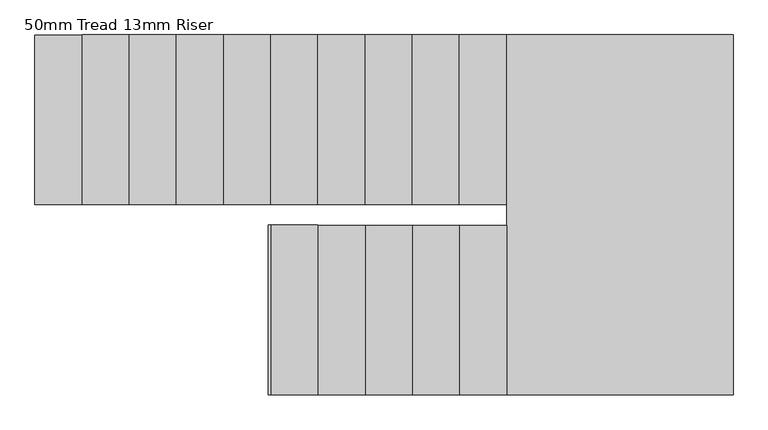
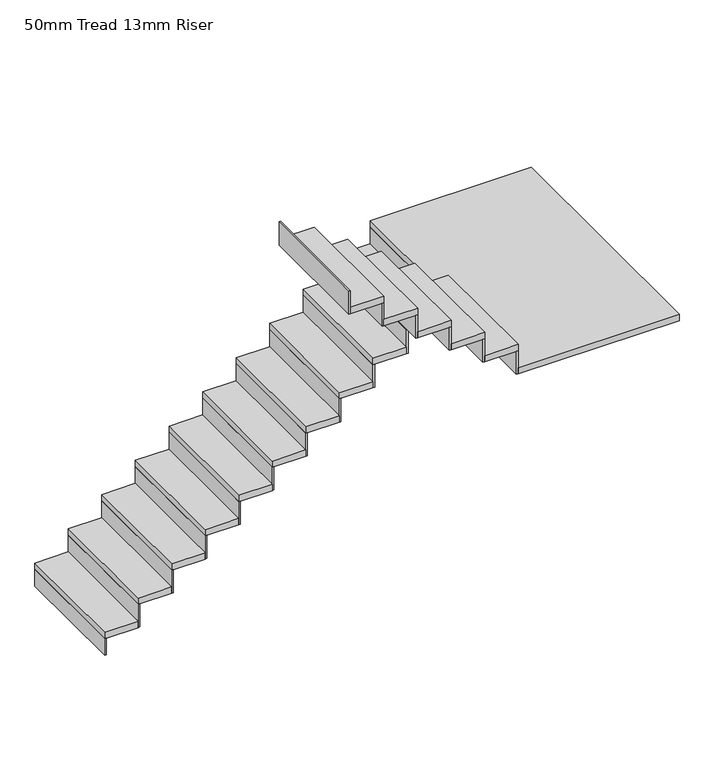
"""IFC4 building model written with IfcOpenShell, lengths in millimetres: stair flight geometry, 50mm Tread 13mm Riser."""

from ifc_helpers import new_model, si_unit, frame, origin, place, context, project, spatial, polyline, outline, extrude, source, transform, mapped, element, save


def stair_flight_50mm_tread_13mm_riser_aed1185b(model_context):
    return source(origin(), model_context, "Body", "SweptSolid", [
        extrude(outline(polyline([(-8706.7253352, 6708.2914588), (-8719.2253352, 6708.2914588), (-8719.2253352, 7608.2914588), (-8706.7253352, 7608.2914588), (-8706.7253352, 6708.2914588)])), frame((0.0, 0.0, 450.0), z_axis=(0.0, 0.0, 1.0), x_axis=(1.0, 0.0, 0.0)), (0.0, 0.0, 1.0), 132.3529412),
        extrude(outline(polyline([(-8469.2253352, 7608.2914588), (-8469.2253352, 6708.2914588), (-8719.2253352, 6708.2914588), (-8719.2253352, 7608.2914588), (-8469.2253352, 7608.2914588)])), frame((0.0, 0.0, 582.3529412), z_axis=(0.0, 0.0, 1.0), x_axis=(1.0, 0.0, 0.0)), (0.0, 0.0, 1.0), 50.0),
        extrude(outline(polyline([(-8456.7253352, 6708.2914588), (-8469.2253352, 6708.2914588), (-8469.2253352, 7608.2914588), (-8456.7253352, 7608.2914588), (-8456.7253352, 6708.2914588)])), frame((0.0, 0.0, 582.3529412), z_axis=(0.0, 0.0, 1.0), x_axis=(1.0, 0.0, 0.0)), (0.0, 0.0, 1.0), 182.3529412),
        extrude(outline(polyline([(-8219.2253352, 7608.2914588), (-8219.2253352, 6708.2914588), (-8469.2253352, 6708.2914588), (-8469.2253352, 7608.2914588), (-8219.2253352, 7608.2914588)])), frame((0.0, 0.0, 764.7058824), z_axis=(0.0, 0.0, 1.0), x_axis=(1.0, 0.0, 0.0)), (0.0, 0.0, 1.0), 50.0),
        extrude(outline(polyline([(-8206.7253352, 6708.2914588), (-8219.2253352, 6708.2914588), (-8219.2253352, 7608.2914588), (-8206.7253352, 7608.2914588), (-8206.7253352, 6708.2914588)])), frame((0.0, 0.0, 764.7058824), z_axis=(0.0, 0.0, 1.0), x_axis=(1.0, 0.0, 0.0)), (0.0, 0.0, 1.0), 182.3529412),
        extrude(outline(polyline([(-7969.2253352, 7608.2914588), (-7969.2253352, 6708.2914588), (-8219.2253352, 6708.2914588), (-8219.2253352, 7608.2914588), (-7969.2253352, 7608.2914588)])), frame((0.0, 0.0, 947.0588235), z_axis=(0.0, 0.0, 1.0), x_axis=(1.0, 0.0, 0.0)), (0.0, 0.0, 1.0), 50.0),
        extrude(outline(polyline([(-7956.7253352, 6708.2914588), (-7969.2253352, 6708.2914588), (-7969.2253352, 7608.2914588), (-7956.7253352, 7608.2914588), (-7956.7253352, 6708.2914588)])), frame((0.0, 0.0, 947.0588235), z_axis=(0.0, 0.0, 1.0), x_axis=(1.0, 0.0, 0.0)), (0.0, 0.0, 1.0), 182.3529412),
        extrude(outline(polyline([(-7719.2253352, 7608.2914588), (-7719.2253352, 6708.2914588), (-7969.2253352, 6708.2914588), (-7969.2253352, 7608.2914588), (-7719.2253352, 7608.2914588)])), frame((0.0, 0.0, 1129.4117647), z_axis=(0.0, 0.0, 1.0), x_axis=(1.0, 0.0, 0.0)), (0.0, 0.0, 1.0), 50.0),
        extrude(outline(polyline([(-7706.7253352, 6708.2914588), (-7719.2253352, 6708.2914588), (-7719.2253352, 7608.2914588), (-7706.7253352, 7608.2914588), (-7706.7253352, 6708.2914588)])), frame((0.0, 0.0, 1129.4117647), z_axis=(0.0, 0.0, 1.0), x_axis=(1.0, 0.0, 0.0)), (0.0, 0.0, 1.0), 182.3529412),
        extrude(outline(polyline([(-7469.2253352, 7608.2914588), (-7469.2253352, 6708.2914588), (-7719.2253352, 6708.2914588), (-7719.2253352, 7608.2914588), (-7469.2253352, 7608.2914588)])), frame((0.0, 0.0, 1311.7647059), z_axis=(0.0, 0.0, 1.0), x_axis=(1.0, 0.0, 0.0)), (0.0, 0.0, 1.0), 50.0),
        extrude(outline(polyline([(-7456.7253352, 6708.2914588), (-7469.2253352, 6708.2914588), (-7469.2253352, 7608.2914588), (-7456.7253352, 7608.2914588), (-7456.7253352, 6708.2914588)])), frame((0.0, 0.0, 1311.7647059), z_axis=(0.0, 0.0, 1.0), x_axis=(1.0, 0.0, 0.0)), (0.0, 0.0, 1.0), 182.3529412),
        extrude(outline(polyline([(-7219.2253352, 7608.2914588), (-7219.2253352, 6708.2914588), (-7469.2253352, 6708.2914588), (-7469.2253352, 7608.2914588), (-7219.2253352, 7608.2914588)])), frame((0.0, 0.0, 1494.1176471), z_axis=(0.0, 0.0, 1.0), x_axis=(1.0, 0.0, 0.0)), (0.0, 0.0, 1.0), 50.0),
        extrude(outline(polyline([(-7206.7253352, 6708.2914588), (-7219.2253352, 6708.2914588), (-7219.2253352, 7608.2914588), (-7206.7253352, 7608.2914588), (-7206.7253352, 6708.2914588)])), frame((0.0, 0.0, 1494.1176471), z_axis=(0.0, 0.0, 1.0), x_axis=(1.0, 0.0, 0.0)), (0.0, 0.0, 1.0), 182.3529412),
        extrude(outline(polyline([(-6969.2253352, 7608.2914588), (-6969.2253352, 6708.2914588), (-7219.2253352, 6708.2914588), (-7219.2253352, 7608.2914588), (-6969.2253352, 7608.2914588)])), frame((0.0, 0.0, 1676.4705882), z_axis=(0.0, 0.0, 1.0), x_axis=(1.0, 0.0, 0.0)), (0.0, 0.0, 1.0), 50.0),
        extrude(outline(polyline([(-6956.7253352, 6708.2914588), (-6969.2253352, 6708.2914588), (-6969.2253352, 7608.2914588), (-6956.7253352, 7608.2914588), (-6956.7253352, 6708.2914588)])), frame((0.0, 0.0, 1676.4705882), z_axis=(0.0, 0.0, 1.0), x_axis=(1.0, 0.0, 0.0)), (0.0, 0.0, 1.0), 182.3529412),
        extrude(outline(polyline([(-6719.2253352, 7608.2914588), (-6719.2253352, 6708.2914588), (-6969.2253352, 6708.2914588), (-6969.2253352, 7608.2914588), (-6719.2253352, 7608.2914588)])), frame((0.0, 0.0, 1858.8235294), z_axis=(0.0, 0.0, 1.0), x_axis=(1.0, 0.0, 0.0)), (0.0, 0.0, 1.0), 50.0),
        extrude(outline(polyline([(-6706.7253352, 6708.2914588), (-6719.2253352, 6708.2914588), (-6719.2253352, 7608.2914588), (-6706.7253352, 7608.2914588), (-6706.7253352, 6708.2914588)])), frame((0.0, 0.0, 1858.8235294), z_axis=(0.0, 0.0, 1.0), x_axis=(1.0, 0.0, 0.0)), (0.0, 0.0, 1.0), 182.3529412),
        extrude(outline(polyline([(-6469.2253352, 7608.2914588), (-6469.2253352, 6708.2914588), (-6719.2253352, 6708.2914588), (-6719.2253352, 7608.2914588), (-6469.2253352, 7608.2914588)])), frame((0.0, 0.0, 2041.1764706), z_axis=(0.0, 0.0, 1.0), x_axis=(1.0, 0.0, 0.0)), (0.0, 0.0, 1.0), 50.0),
        extrude(outline(polyline([(-6456.7253352, 6708.2914588), (-6469.2253352, 6708.2914588), (-6469.2253352, 7608.2914588), (-6456.7253352, 7608.2914588), (-6456.7253352, 6708.2914588)])), frame((0.0, 0.0, 2041.1764706), z_axis=(0.0, 0.0, 1.0), x_axis=(1.0, 0.0, 0.0)), (0.0, 0.0, 1.0), 182.3529412),
        extrude(outline(polyline([(-6219.2253352, 7608.2914588), (-6219.2253352, 6708.2914588), (-6469.2253352, 6708.2914588), (-6469.2253352, 7608.2914588), (-6219.2253352, 7608.2914588)])), frame((0.0, 0.0, 2223.5294118), z_axis=(0.0, 0.0, 1.0), x_axis=(1.0, 0.0, 0.0)), (0.0, 0.0, 1.0), 50.0),
        extrude(outline(polyline([(-6206.7253352, 6708.2914588), (-6219.2253352, 6708.2914588), (-6219.2253352, 7608.2914588), (-6206.7253352, 7608.2914588), (-6206.7253352, 6708.2914588)])), frame((0.0, 0.0, 2223.5294118), z_axis=(0.0, 0.0, 1.0), x_axis=(1.0, 0.0, 0.0)), (0.0, 0.0, 1.0), 182.3529412),
        extrude(outline(polyline([(-6219.2253352, 5698.2914588), (-6219.2253352, 6598.2914588), (-6219.2253352, 6708.2914588), (-6219.2253352, 7608.2914588), (-5019.2253352, 7608.2914588), (-5019.2253352, 5698.2914588), (-6219.2253352, 5698.2914588)])), frame((0.0, 0.0, 2405.8823529), z_axis=(0.0, 0.0, 1.0), x_axis=(1.0, 0.0, 0.0)), (0.0, 0.0, 1.0), 50.0),
        extrude(outline(polyline([(-6231.7253352, 6598.2914588), (-6219.2253352, 6598.2914588), (-6219.2253352, 5698.2914588), (-6231.7253352, 5698.2914588), (-6231.7253352, 6598.2914588)])), frame((0.0, 0.0, 2405.8823529), z_axis=(0.0, 0.0, 1.0), x_axis=(1.0, 0.0, 0.0)), (0.0, 0.0, 1.0), 182.3529412),
        extrude(outline(polyline([(-6469.2253352, 5698.2914588), (-6469.2253352, 6598.2914588), (-6219.2253352, 6598.2914588), (-6219.2253352, 5698.2914588), (-6469.2253352, 5698.2914588)])), frame((0.0, 0.0, 2588.2352941), z_axis=(0.0, 0.0, 1.0), x_axis=(1.0, 0.0, 0.0)), (0.0, 0.0, 1.0), 50.0),
        extrude(outline(polyline([(-6481.7253352, 6598.2914588), (-6469.2253352, 6598.2914588), (-6469.2253352, 5698.2914588), (-6481.7253352, 5698.2914588), (-6481.7253352, 6598.2914588)])), frame((0.0, 0.0, 2588.2352941), z_axis=(0.0, 0.0, 1.0), x_axis=(1.0, 0.0, 0.0)), (0.0, 0.0, 1.0), 182.3529412),
        extrude(outline(polyline([(-6719.2253352, 5698.2914588), (-6719.2253352, 6598.2914588), (-6469.2253352, 6598.2914588), (-6469.2253352, 5698.2914588), (-6719.2253352, 5698.2914588)])), frame((0.0, 0.0, 2770.5882353), z_axis=(0.0, 0.0, 1.0), x_axis=(1.0, 0.0, 0.0)), (0.0, 0.0, 1.0), 50.0),
        extrude(outline(polyline([(-6731.7253352, 6598.2914588), (-6719.2253352, 6598.2914588), (-6719.2253352, 5698.2914588), (-6731.7253352, 5698.2914588), (-6731.7253352, 6598.2914588)])), frame((0.0, 0.0, 2770.5882353), z_axis=(0.0, 0.0, 1.0), x_axis=(1.0, 0.0, 0.0)), (0.0, 0.0, 1.0), 182.3529412),
        extrude(outline(polyline([(-6969.2253352, 5698.2914588), (-6969.2253352, 6598.2914588), (-6719.2253352, 6598.2914588), (-6719.2253352, 5698.2914588), (-6969.2253352, 5698.2914588)])), frame((0.0, 0.0, 2952.9411765), z_axis=(0.0, 0.0, 1.0), x_axis=(1.0, 0.0, 0.0)), (0.0, 0.0, 1.0), 50.0),
        extrude(outline(polyline([(-6981.7253352, 6598.2914588), (-6969.2253352, 6598.2914588), (-6969.2253352, 5698.2914588), (-6981.7253352, 5698.2914588), (-6981.7253352, 6598.2914588)])), frame((0.0, 0.0, 2952.9411765), z_axis=(0.0, 0.0, 1.0), x_axis=(1.0, 0.0, 0.0)), (0.0, 0.0, 1.0), 182.3529412),
        extrude(outline(polyline([(-7219.2253352, 5698.2914588), (-7219.2253352, 6598.2914588), (-6969.2253352, 6598.2914588), (-6969.2253352, 5698.2914588), (-7219.2253352, 5698.2914588)])), frame((0.0, 0.0, 3135.2941176), z_axis=(0.0, 0.0, 1.0), x_axis=(1.0, 0.0, 0.0)), (0.0, 0.0, 1.0), 50.0),
        extrude(outline(polyline([(-7231.7253352, 6598.2914588), (-7219.2253352, 6598.2914588), (-7219.2253352, 5698.2914588), (-7231.7253352, 5698.2914588), (-7231.7253352, 6598.2914588)])), frame((0.0, 0.0, 3135.2941176), z_axis=(0.0, 0.0, 1.0), x_axis=(1.0, 0.0, 0.0)), (0.0, 0.0, 1.0), 182.3529412),
        extrude(outline(polyline([(-7481.7253352, 6598.2914588), (-7469.2253352, 6598.2914588), (-7469.2253352, 5698.2914588), (-7481.7253352, 5698.2914588), (-7481.7253352, 6598.2914588)])), frame((0.0, 0.0, 3317.6470588), z_axis=(0.0, 0.0, 1.0), x_axis=(1.0, 0.0, 0.0)), (0.0, 0.0, 1.0), 182.3529412),
        extrude(outline(polyline([(-7469.2253352, 5698.2914588), (-7469.2253352, 6598.2914588), (-7219.2253352, 6598.2914588), (-7219.2253352, 5698.2914588), (-7469.2253352, 5698.2914588)])), frame((0.0, 0.0, 3317.6470588), z_axis=(0.0, 0.0, 1.0), x_axis=(1.0, 0.0, 0.0)), (0.0, 0.0, 1.0), 50.0),
    ])


if __name__ == "__main__":
    model = new_model("IFC4")
    model_context = context("Model", 3, world=origin())
    ifc_project = project(units=[si_unit("LENGTHUNIT", "METRE", prefix="MILLI")], contexts=[model_context])
    site = spatial("IfcSite", under=ifc_project)
    building = spatial("IfcBuilding", under=site)
    placement = place(None, origin())
    stair_flight_50mm_tread_13mm_riser_shape = stair_flight_50mm_tread_13mm_riser_aed1185b(model_context)
    element("IfcStairFlight", 1, ObjectType="50mm Tread 13mm Riser", at=placement, inside=building, context=model_context, shape_type="MappedRepresentation", body=[
        mapped(stair_flight_50mm_tread_13mm_riser_shape, transform((0.0, 0.0, 0.0), x_axis=(1.0, 0.0, 0.0), y_axis=(0.0, 1.0, 0.0), z_axis=(0.0, 0.0, 1.0))),
    ])
    save(model, "model.ifc")
